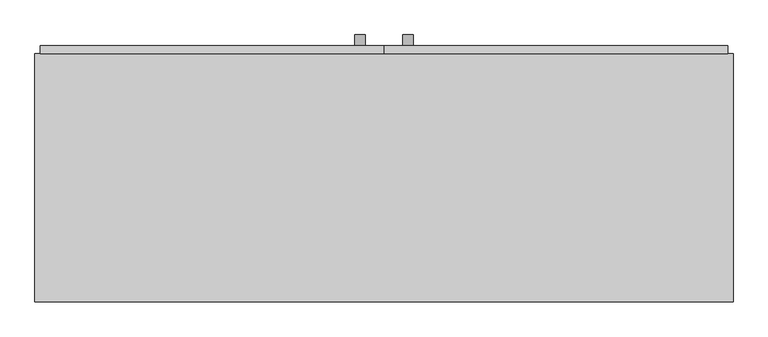
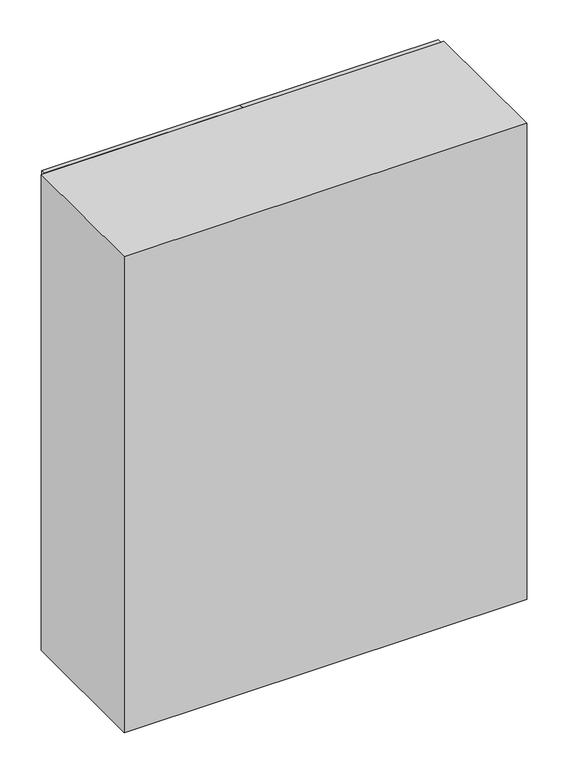
"""IFC4 building model written with IfcOpenShell, lengths in millimetres: furniture geometry, Armario dormitorio : ARMARIO DORM_PABLO."""

from ifc_helpers import new_model, si_unit, point, frame, frame_2d, origin, origin_with_axes, place, context, project, spatial, polyline, circle_curve, trimmed, segment, composite_curve, outline, extrude, source, transform, mapped, element, save


def furniture_bc266251(model_context):
    return source(origin(), model_context, "Body", "SweptSolid", [
        extrude(outline(composite_curve([segment(trimmed(circle_curve(frame_2d((1100.0, -55.0)), 12.5), [point((1100.0, -67.5))], [point((1100.0, -42.5))], False, "CARTESIAN"), True, "CONTINUOUS"), segment(trimmed(circle_curve(frame_2d((1100.0, -55.0)), 12.5), [point((1100.0, -42.5))], [point((1100.0, -67.5))], False, "CARTESIAN"), True, "CONTINUOUS")], self_intersect=False)), frame((0.0, 588.0, 0.0), z_axis=(0.0, 1.0, 0.0), x_axis=(0.0, 0.0, 1.0)), (0.0, 0.0, 1.0), 25.0),
        extrude(outline(composite_curve([segment(trimmed(circle_curve(frame_2d((1100.0, 55.0)), 12.5), [point((1100.0, 42.5))], [point((1100.0, 67.5))], False, "CARTESIAN"), True, "CONTINUOUS"), segment(trimmed(circle_curve(frame_2d((1100.0, 55.0)), 12.5), [point((1100.0, 67.5))], [point((1100.0, 42.5))], False, "CARTESIAN"), True, "CONTINUOUS")], self_intersect=False)), frame((0.0, 588.0, 0.0), z_axis=(0.0, 1.0, 0.0), x_axis=(0.0, 0.0, 1.0)), (0.0, 0.0, 1.0), 25.0),
        extrude(outline(polyline([(0.0, 570.0), (0.0, 588.0), (787.5, 588.0), (787.5, 570.0), (0.0, 570.0)])), frame((0.0, 0.0, 18.0), z_axis=(0.0, 0.0, 1.0), x_axis=(1.0, 0.0, 0.0)), (0.0, 0.0, 1.0), 1982.0),
        extrude(outline(polyline([(0.0, 570.0), (-787.5, 570.0), (-787.5, 588.0), (0.0, 588.0), (0.0, 570.0)])), frame((0.0, 0.0, 18.0), z_axis=(0.0, 0.0, 1.0), x_axis=(1.0, 0.0, 0.0)), (0.0, 0.0, 1.0), 1982.0),
        extrude(outline(polyline([(800.0, 0.0), (-800.0, 0.0), (-800.0, 570.0), (800.0, 570.0), (800.0, 0.0)])), origin_with_axes(), (0.0, 0.0, 1.0), 2000.0),
    ])


if __name__ == "__main__":
    model = new_model("IFC4")
    model_context = context("Model", 3, world=origin())
    ifc_project = project(units=[si_unit("LENGTHUNIT", "METRE", prefix="MILLI")], contexts=[model_context])
    site = spatial("IfcSite", under=ifc_project)
    building = spatial("IfcBuilding", under=site)
    placement = place(None, origin())
    furniture_shape = furniture_bc266251(model_context)
    element("IfcFurniture", 1, ObjectType="Armario dormitorio : ARMARIO DORM_PABLO", at=placement, inside=building, context=model_context, shape_type="MappedRepresentation", body=[
        mapped(furniture_shape, transform((0.0, 0.0, 0.0), x_axis=(1.0, 0.0, 0.0), y_axis=(0.0, 1.0, 0.0), z_axis=(0.0, 0.0, 1.0))),
    ])
    save(model, "model.ifc")

# Revit data of these elements
# Type "Armario dormitorio : ARMARIO DORM_PABLO"
#   Anchura = 1.60 m
#   Altura = 2.00 m
#   Profundidad = 0.57 m
#   Material de armario = none
#   Default Elevation = 0
# Element 1 (IfcFurniture, "Armario dormitorio : ARMARIO DORM_PABLO")
#   Materials on its faces: "Madera - Listel"
# Materials
#   "Madera - Listel": class "Madera", colour RGB 210 180 110, transparency 0, Cost = 0
